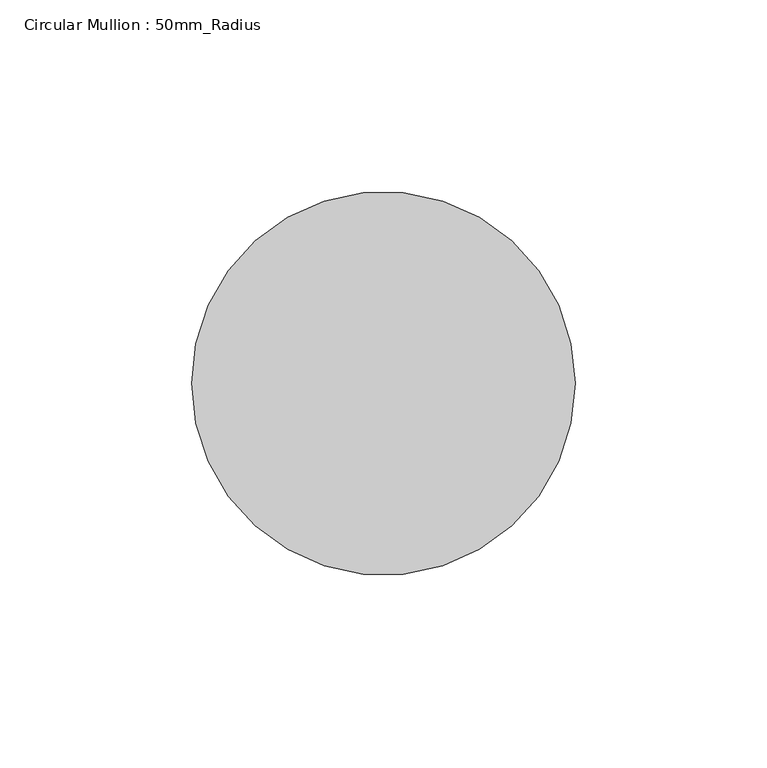
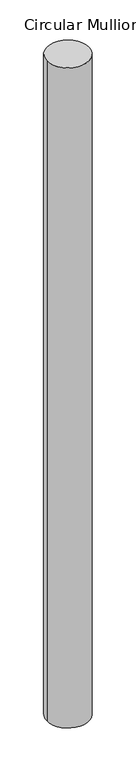
"""IFC4 building model written with IfcOpenShell, lengths in millimetres: member geometry, Circular Mullion : 50mm_Radius."""

import ifcopenshell
import ifcopenshell.guid

model = None  # the IFC model being written
_history = None  # IfcOwnerHistory: only IFC2X3 demands one
_inside = {}  # id of a spatial element -> (the spatial element, [elements in it])
_under = {}  # id of a project, library or spatial element -> (it, [spatial elements below it])
_declared = {}  # id of a project -> (the project, [libraries it declares])
_typed = {}  # id of a type object -> (the type object, [elements of that type])
_made_of = {}  # id of a material, layer set ... -> (it, [elements and type objects made of it])


def new_model(schema):
    """Start an empty IFC model of exactly this schema.

    Asked for "IFC4X3", IfcOpenShell would pick the latest addendum, in which some entities
    have other attributes; the version numbers below select the first issue.
    IFC2X3 requires an IfcOwnerHistory on every rooted entity: one is made here for all.
    """
    global model, _history
    if schema == "IFC4X3":
        model = ifcopenshell.file(schema_version=(4, 3, 0, 0))
    else:
        model = ifcopenshell.file(schema=schema)
    _inside.clear()
    _under.clear()
    _declared.clear()
    _typed.clear()
    _made_of.clear()
    _history = None
    if model.schema == "IFC2X3":
        org = make("IfcOrganization", Name="unknown")
        user = make(
            "IfcPersonAndOrganization",
            ThePerson=make("IfcPerson", FamilyName="unknown"),
            TheOrganization=org,
        )
        app = make(
            "IfcApplication",
            ApplicationDeveloper=org,
            Version="unknown",
            ApplicationFullName="unknown",
            ApplicationIdentifier="unknown",
        )
        _history = make(
            "IfcOwnerHistory",
            OwningUser=user,
            OwningApplication=app,
            ChangeAction="ADDED",
            CreationDate=0,
        )
    return model


def make(cls, **values):
    """One entity of the class cls with the attributes given. An attribute that is None is left unset."""
    return model.create_entity(
        cls, **{name: value for name, value in values.items() if value is not None}
    )


def rooted(cls, **values):
    """An entity with a GlobalId (a new one), such as an element, a storey or a relation."""
    return make(cls, GlobalId=ifcopenshell.guid.new(), OwnerHistory=_history, **values)


def si_unit(unit_type, name, prefix=None):
    """IfcSIUnit, for example si_unit("LENGTHUNIT", "METRE", prefix="MILLI")."""
    return make("IfcSIUnit", UnitType=unit_type, Prefix=prefix, Name=name)


def assignment(units):
    """IfcUnitAssignment: the units of a project."""
    return None if units is None else make("IfcUnitAssignment", Units=units)


def point(xyz):
    """IfcCartesianPoint."""
    return None if xyz is None else make("IfcCartesianPoint", Coordinates=xyz)


def direction(xyz):
    """IfcDirection."""
    return None if xyz is None else make("IfcDirection", DirectionRatios=xyz)


def frame(location, z_axis=None, x_axis=None):
    """IfcAxis2Placement3D, a coordinate frame: its origin and axes. An axis left out is left unset."""
    return make(
        "IfcAxis2Placement3D",
        Location=point(location),
        Axis=direction(z_axis),
        RefDirection=direction(x_axis),
    )


def frame_2d(location, x_axis=None):
    """IfcAxis2Placement2D, a coordinate frame in the plane: its origin and x axis."""
    return make(
        "IfcAxis2Placement2D", Location=point(location), RefDirection=direction(x_axis)
    )


def origin():
    """The frame at (0, 0, 0) with its axes left unset."""
    return frame((0.0, 0.0, 0.0))


def origin_2d():
    """The frame at (0, 0) in the plane with its x axis left unset."""
    return frame_2d((0.0, 0.0))


def place(relative_to, where):
    """IfcLocalPlacement: puts the frame where relative to a parent placement (None: the world)."""
    return make(
        "IfcLocalPlacement", PlacementRelTo=relative_to, RelativePlacement=where
    )


def context(
    kind, dimensions, precision=None, world=None, true_north=None, identifier=None
):
    """IfcGeometricRepresentationContext, for example the 3D "Model" context."""
    return make(
        "IfcGeometricRepresentationContext",
        ContextIdentifier=identifier,
        ContextType=kind,
        CoordinateSpaceDimension=dimensions,
        Precision=precision,
        WorldCoordinateSystem=world,
        TrueNorth=true_north,
    )


def project(units=None, contexts=None):
    """IfcProject with its units and contexts."""
    return rooted(
        "IfcProject",
        Name="project",
        RepresentationContexts=contexts,
        UnitsInContext=assignment(units),
    )


def spatial(cls, under=None, at=None, **own):
    """A site, building, storey or space (cls), placed at a placement, below another one or the project."""
    s = rooted(cls, ObjectPlacement=at, **own)
    if under is not None:
        _under.setdefault(under.id(), (under, []))[1].append(s)
    return s


def circle_curve(where, radius):
    """IfcCircle in the frame where."""
    return make("IfcCircle", Position=where, Radius=radius)


def trimmed(basis, trim1, trim2, sense, master):
    """IfcTrimmedCurve: the piece of a basis curve between two trims."""
    return make(
        "IfcTrimmedCurve",
        BasisCurve=basis,
        Trim1=trim1,
        Trim2=trim2,
        SenseAgreement=sense,
        MasterRepresentation=master,
    )


def segment(curve, same_sense, transition):
    """IfcCompositeCurveSegment."""
    return make(
        "IfcCompositeCurveSegment",
        Transition=transition,
        SameSense=same_sense,
        ParentCurve=curve,
    )


def composite_curve(segments, self_intersect=None):
    """IfcCompositeCurve: segments joined end to end."""
    return make("IfcCompositeCurve", Segments=segments, SelfIntersect=self_intersect)


def outline(outer, holes=None, kind="AREA"):
    """IfcArbitraryClosedProfileDef: a profile drawn as a closed curve; with holes, ...WithVoids."""
    if holes is None:
        return make("IfcArbitraryClosedProfileDef", ProfileType=kind, OuterCurve=outer)
    return make(
        "IfcArbitraryProfileDefWithVoids",
        ProfileType=kind,
        OuterCurve=outer,
        InnerCurves=holes,
    )


def extrude(swept, where, along, depth):
    """IfcExtrudedAreaSolid: the profile swept, set in the frame where, extruded along a direction by depth."""
    return make(
        "IfcExtrudedAreaSolid",
        SweptArea=swept,
        Position=where,
        ExtrudedDirection=direction(along),
        Depth=depth,
    )


def shape(context_of_items, identifier, shape_type, items):
    """IfcShapeRepresentation: the items that make up one representation, for example the "Body"."""
    return make(
        "IfcShapeRepresentation",
        ContextOfItems=context_of_items,
        RepresentationIdentifier=identifier,
        RepresentationType=shape_type,
        Items=items,
    )


def source(mapping_origin, context_of_items, identifier, shape_type, items):
    """IfcRepresentationMap: a shape defined once, which mapped items show again and again."""
    return make(
        "IfcRepresentationMap",
        MappingOrigin=mapping_origin,
        MappedRepresentation=shape(context_of_items, identifier, shape_type, items),
    )


def transform(
    local_origin,
    x_axis=None,
    y_axis=None,
    z_axis=None,
    scale=None,
    scale2=None,
    scale3=None,
    uniform=True,
):
    """IfcCartesianTransformationOperator3D, or its non-uniform kind. x_axis, y_axis, z_axis: its Axis1, 2, 3."""
    if uniform:
        return make(
            "IfcCartesianTransformationOperator3D",
            Axis1=direction(x_axis),
            Axis2=direction(y_axis),
            LocalOrigin=point(local_origin),
            Scale=scale,
            Axis3=direction(z_axis),
        )
    return make(
        "IfcCartesianTransformationOperator3DnonUniform",
        Axis1=direction(x_axis),
        Axis2=direction(y_axis),
        LocalOrigin=point(local_origin),
        Scale=scale,
        Axis3=direction(z_axis),
        Scale2=scale2,
        Scale3=scale3,
    )


def mapped(mapping_source, mapping_target):
    """IfcMappedItem: shows the shape of a source again, moved by a transform."""
    return make(
        "IfcMappedItem", MappingSource=mapping_source, MappingTarget=mapping_target
    )


def made_of(thing, what):
    """Note that an element or type object is made of a material, layer set ...; save() writes the relation."""
    if what is not None:
        _made_of.setdefault(what.id(), (what, []))[1].append(thing)
    return thing


def element(
    cls,
    number,
    at=None,
    inside=None,
    cuts=None,
    type_object=None,
    material=None,
    context=None,
    identifier="Body",
    shape_type=None,
    held_by="IfcProductDefinitionShape",
    body=None,
    shapes=None,
    **own,
):
    """One element of the class cls, such as IfcWall. Its Tag is "e" and its number.

    at: its placement. inside: the storey or other place that contains it. cuts: it is an
    opening in that element (IfcRelVoidsElement). A single representation is given by context,
    identifier, shape_type and body (its items); several are given by shapes. held_by: the class
    of the entity that holds the representations. save() writes the other relations.
    """
    e = rooted(cls, Tag="e%d" % number, ObjectPlacement=at, **own)
    if body is not None:
        shapes = [shape(context, identifier, shape_type, body)]
    if shapes is not None:
        e.Representation = make(held_by, Representations=shapes)
    if inside is not None:
        _inside.setdefault(inside.id(), (inside, []))[1].append(e)
    if cuts is not None:
        rooted(
            "IfcRelVoidsElement", RelatingBuildingElement=cuts, RelatedOpeningElement=e
        )
    if type_object is not None:
        _typed.setdefault(type_object.id(), (type_object, []))[1].append(e)
    return made_of(e, material)


def aggregate(whole, parts):
    """IfcRelAggregates: a whole, such as a stair, and the parts it consists of."""
    return rooted("IfcRelAggregates", RelatingObject=whole, RelatedObjects=parts)


def save(model, path):
    """Write the relations noted so far, then the file.

    IfcRelAggregates (storeys below a building ...), IfcRelContainedInSpatialStructure (elements
    in a storey), IfcRelDefinesByType, IfcRelAssociatesMaterial and IfcRelDeclares: one each for
    every whole, place, type object, material and project.
    """
    for whole, parts in _under.values():
        aggregate(whole, parts)
    for where, things in _inside.values():
        rooted(
            "IfcRelContainedInSpatialStructure",
            RelatedElements=things,
            RelatingStructure=where,
        )
    for kind, things in _typed.values():
        rooted("IfcRelDefinesByType", RelatedObjects=things, RelatingType=kind)
    for what, things in _made_of.values():
        rooted("IfcRelAssociatesMaterial", RelatedObjects=things, RelatingMaterial=what)
    for by, libraries in _declared.values():
        rooted("IfcRelDeclares", RelatingContext=by, RelatedDefinitions=libraries)
    model.write(path)


def circular_mullion_50mm_radius_be99d508(model_context):
    return source(origin(), model_context, "Body", "SweptSolid", [
        extrude(outline(composite_curve([segment(trimmed(circle_curve(origin_2d(), 50.0), [point((50.0, 0.0))], [point((-50.0, 0.0))], False, "CARTESIAN"), True, "CONTINUOUS"), segment(trimmed(circle_curve(origin_2d(), 50.0), [point((-50.0, 0.0))], [point((50.0, 0.0))], False, "CARTESIAN"), True, "CONTINUOUS")], self_intersect=False)), frame((0.0, 0.0, -1655.0000003), z_axis=(0.0, 0.0, 1.0), x_axis=(1.0, 0.0, 0.0)), (0.0, 0.0, 1.0), 1655.0000003),
    ])


if __name__ == "__main__":
    model = new_model("IFC4")
    model_context = context("Model", 3, world=origin())
    ifc_project = project(units=[si_unit("LENGTHUNIT", "METRE", prefix="MILLI")], contexts=[model_context])
    site = spatial("IfcSite", under=ifc_project)
    building = spatial("IfcBuilding", under=site)
    placement = place(None, origin())
    circular_mullion_50mm_radius_shape = circular_mullion_50mm_radius_be99d508(model_context)
    element("IfcMember", 1, ObjectType="Circular Mullion : 50mm_Radius", at=placement, inside=building, context=model_context, shape_type="MappedRepresentation", body=[
        mapped(circular_mullion_50mm_radius_shape, transform((0.0, 0.0, 0.0), x_axis=(1.0, 0.0, 0.0), y_axis=(0.0, 1.0, 0.0), z_axis=(0.0, 0.0, 1.0))),
    ])
    save(model, "model.ifc")

# Revit data of these elements
# Type "Circular Mullion : 50mm_Radius"
#   Keynote = "H11"
#   built-in parameter 1007350 = 0.164042 (stored number, unit not read)
# Element 1 (IfcMember, "Circular Mullion : 50mm_Radius")
#   Materials on its faces: "Aluminium"
# Materials
#   "Aluminium": class "Metal", colour RGB 247 247 247, transparency 0, Description = "Aluminium 6061", Cost = 0
